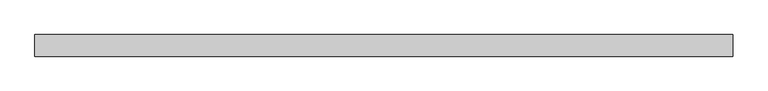
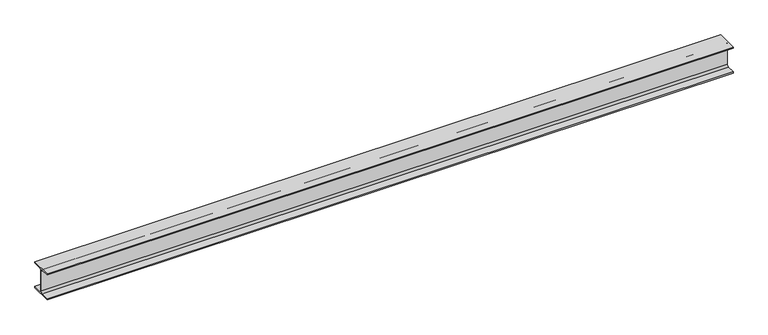
"""IFC4 building model written with IfcOpenShell, lengths in millimetres: beam geometry, 0912_Steel Framing_H-KSD3502 : H_SB_AR_S02_H-194x150x6x9_Platform."""

from ifc_helpers import new_model, si_unit, point, frame, frame_2d, origin, place, context, project, spatial, polyline, circle_curve, trimmed, segment, composite_curve, outline, extrude, source, transform, mapped, element, save


def beam_42108b3c(model_context):
    return source(origin(), model_context, "Body", "SweptSolid", [
        extrude(outline(composite_curve([segment(polyline([(75.0, -88.0), (75.0, -97.0), (-75.0, -97.0), (-75.0, -88.0), (-16.0, -88.0)]), True, "CONTINUOUS"), segment(trimmed(circle_curve(frame_2d((-16.0, -75.0)), 13.0), [point((-16.0, -88.0))], [point((-3.0, -75.0))], True, "CARTESIAN"), True, "CONTINUOUS"), segment(polyline([(-3.0, -75.0), (-3.0, 75.0)]), True, "CONTINUOUS"), segment(trimmed(circle_curve(frame_2d((-16.0, 75.0)), 13.0), [point((-3.0, 75.0))], [point((-16.0, 88.0))], True, "CARTESIAN"), True, "CONTINUOUS"), segment(polyline([(-16.0, 88.0), (-75.0, 88.0), (-75.0, 97.0), (75.0, 97.0), (75.0, 88.0), (16.0, 88.0)]), True, "CONTINUOUS"), segment(trimmed(circle_curve(frame_2d((16.0, 75.0)), 13.0), [point((16.0, 88.0))], [point((3.0, 75.0))], True, "CARTESIAN"), True, "CONTINUOUS"), segment(polyline([(3.0, 75.0), (3.0, -75.0)]), True, "CONTINUOUS"), segment(trimmed(circle_curve(frame_2d((16.0, -75.0)), 13.0), [point((3.0, -75.0))], [point((16.0, -88.0))], True, "CARTESIAN"), True, "CONTINUOUS"), segment(polyline([(16.0, -88.0), (75.0, -88.0)]), True, "CONTINUOUS")], self_intersect=False)), frame((-2430.7698995, 0.0, 0.0), z_axis=(1.0, 0.0, 0.0), x_axis=(0.0, 1.0, 0.0)), (0.0, 0.0, 1.0), 4837.187492),
    ])


if __name__ == "__main__":
    model = new_model("IFC4")
    model_context = context("Model", 3, world=origin())
    ifc_project = project(units=[si_unit("LENGTHUNIT", "METRE", prefix="MILLI")], contexts=[model_context])
    site = spatial("IfcSite", under=ifc_project)
    building = spatial("IfcBuilding", under=site)
    placement = place(None, origin())
    beam_shape = beam_42108b3c(model_context)
    element("IfcBeam", 1, ObjectType="0912_Steel Framing_H-KSD3502 : H_SB_AR_S02_H-194x150x6x9_Platform", at=placement, inside=building, context=model_context, shape_type="MappedRepresentation", body=[
        mapped(beam_shape, transform((0.0, 0.0, 0.0), x_axis=(1.0, 0.0, 0.0), y_axis=(0.0, 1.0, 0.0), z_axis=(0.0, 0.0, 1.0))),
    ])
    save(model, "model.ifc")

# Revit data of these elements
# Type "0912_Steel Framing_H-KSD3502 : H_SB_AR_S02_H-194x150x6x9_Platform"
#   H_Q'ty Cal Type Tag = "SB-Q2"
#   H_WM Code_1 = "S01AA073-00001 |  | TON | Main Steel Structure Fabrication Work | Shelter/Building | Medium Steel - Standard |  |  |  |  |  |  | Material: (   ) | (90)KG/M>Weight≥(30)KG/M | S01AA073-00001 Main Steel Structure Fabrication Work Shelter/Building Medium Steel - Standard         | - Material: ( ASTM A36 )\n- (90)KG/M>Weight≥(30)KG/M"
#   H_WM Code_2 = "S03AA083-00001 |  | TON | Main Steel Structure Erection Work | Shelter/Building | Medium Steel |  |  |  |  |  |  | Material: (   ) | S03AA083-00001 Main Steel Structure Erection Work Shelter/Building Medium Steel         | - Material: ( ASTM A36 )"
#   H_WM Code_3 = "S01AA009-00001 |  | TON | Main Steel Structure Fabrication Work | Shelter/Building | Plates - Gusset, Stiffener, ETC | Material: (   ) | S01AA009-00001 Main Steel Structure Fabrication Work Shelter/Building Plates - Gusset, Stiffener, ETC         |"
#   H_WM Code_4 = "S41AA051-00001 |  | M2 | Steel Structure Paint Work | Shelter/Building | for Non-Fireproofed Steel Surface |  |  |  |  |  |  | Material: (   ) | S41AA051-00001 Steel Structure Paint Work Shelter/Building for Non-Fireproofed Steel Surface         |"
#   Width = 15.0 cm
#   Web Thickness = 0.6 cm
#   Web Fillet = 1.3 cm
#   Warping Constant = 43316.0 cm⁶
#   W = 0
#   Torsional Moment of Inertia = 8.622 cm⁴
#   Section Area = 39.01 cm²
#   Plastic Modulus weak axis = 104.0 cm³
#   Plastic Modulus strong axis = 309.0 cm³
#   Perimeter = 0.95 m²/m
#   Nominal Weight = 30.60 kgf/m
#   Moment of Inertia weak axis = 507.00 cm⁴
#   Moment of Inertia strong axis = 2690.00 cm⁴
#   Height = 19.4 cm
#   Flange Thickness = 0.9 cm
#   Elastic Modulus weak axis = 67.6 cm³
#   Elastic Modulus strong axis = 277.0 cm³
#   Centroid Vertical = 9.7 cm
#   Centroid Horizontal = 7.5 cm
#   Ix = 26900000
#   Length [instance default] = 1524 mm
#   Zx = 309000
#   b = 150 mm
#   h = 194 mm
#   r = 13 mm
#   s = 6 mm
#   t = 9 mm
#   A = 0.003901 m²
#   Structural Material [instance default] = Steel, 45-345
#   Assembly Code = ""
# Element 1 (IfcBeam, "0912_Steel Framing_H-KSD3502 : H_SB_AR_S02_H-194x150x6x9_Platform")
#   Materials on its faces: "Steel, 45-345"
# Materials
#   "Steel, 45-345": class "Metal", colour RGB 189 187 185, transparency 0, Description = "Steel 345 MPa", Cost = 0
